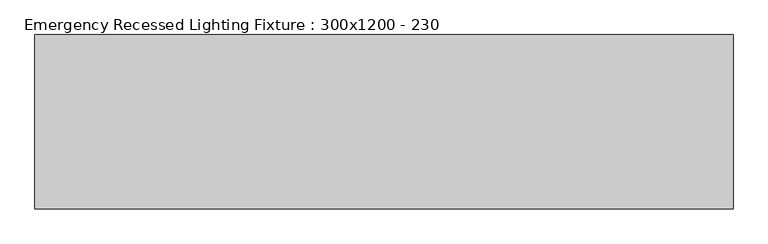
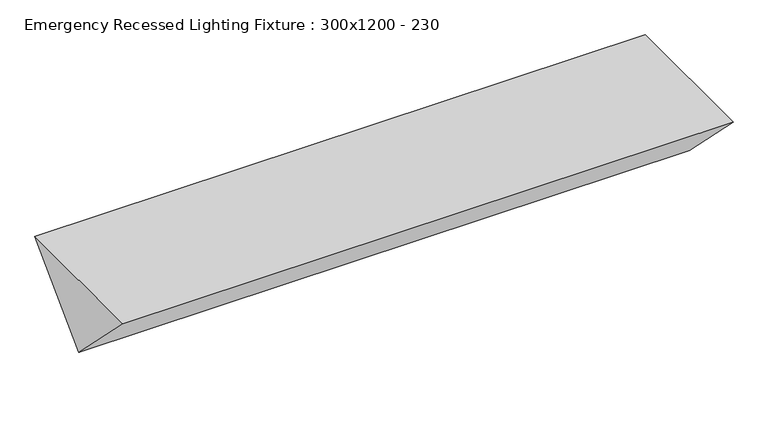
"""IFC4 building model written with IfcOpenShell, lengths in millimetres: light fixture geometry, Emergency Recessed Lighting Fixture : 300x1200 - 230."""

from ifc_helpers import new_model, si_unit, frame, origin, place, context, project, spatial, polyline, outline, extrude, source, transform, mapped, element, save


def emergency_recessed_lighting_fixture_300x1200_230_e46e8774(model_context):
    return source(origin(), model_context, "Body", "SweptSolid", [
        extrude(outline(polyline([(-300.0, 0.0), (0.0, 0.0), (-150.0, -150.0), (-300.0, 0.0)])), frame((0.0, 0.0, 0.0), z_axis=(1.0, 0.0, 0.0), x_axis=(0.0, 1.0, 0.0)), (0.0, 0.0, 1.0), 1200.0),
    ])


if __name__ == "__main__":
    model = new_model("IFC4")
    model_context = context("Model", 3, world=origin())
    ifc_project = project(units=[si_unit("LENGTHUNIT", "METRE", prefix="MILLI")], contexts=[model_context])
    site = spatial("IfcSite", under=ifc_project)
    building = spatial("IfcBuilding", under=site)
    placement = place(None, origin())
    emergency_recessed_lighting_fixture_300x1200_230_shape = emergency_recessed_lighting_fixture_300x1200_230_e46e8774(model_context)
    element("IfcLightFixture", 1, ObjectType="Emergency Recessed Lighting Fixture : 300x1200 - 230", at=placement, inside=building, context=model_context, shape_type="MappedRepresentation", body=[
        mapped(emergency_recessed_lighting_fixture_300x1200_230_shape, transform((0.0, 0.0, 0.0), x_axis=(1.0, 0.0, 0.0), y_axis=(0.0, 1.0, 0.0), z_axis=(0.0, 0.0, 1.0))),
    ])
    save(model, "model.ifc")

# Revit data of these elements
# Type "Emergency Recessed Lighting Fixture : 300x1200 - 230"
#   Photometric Web File = "1x42A12.ies"
#   Width = 300 mm
#   Wattage = 64 W
#   built-in parameter 1150110 = 1 (stored number, unit not read)
#   built-in parameter 1150109 = 1 (stored number, unit not read)
#   built-in parameter 1150113 = 1 (stored number, unit not read)
#   Tilt Angle = -90.00°
#   Normal Voltage = 230 V
#   Lumens = 5699.84 lm
#   built-in parameter 1114217 = 0.88 (stored number, unit not read)
#   built-in parameter 1150115 = 1 (stored number, unit not read)
#   built-in parameter 1150105 = 453.579 (stored number, unit not read)
#   Length = 1200 mm
#   built-in parameter 1150112 = 1 (stored number, unit not read)
#   built-in parameter 1150114 = 1 (stored number, unit not read)
#   built-in parameter 1150107 = 4230 (stored number, unit not read)
#   built-in parameter 1150106 = 4.53579 (stored number, unit not read)
#   Emit from Rectangle Width = 300 mm
#   Emit from Rectangle Length = 1200 mm
#   Emergency Voltage = 230 V
#   Emergency Load = 32 VA
#   built-in parameter 1150104 = 8.27394 (stored number, unit not read)
#   Depth = 150 mm
#   Default Elevation = 2000 mm
#   built-in parameter 1114218 = 0.88 (stored number, unit not read)
#   built-in parameter 1150133 = 10 (stored number, unit not read)
#   Apparent Load = 64 VA
#   built-in parameter 1150134 = 8
#   built-in parameter 1150137 = 1
#   Color Filter = 16777215
#   built-in parameter 1140040 [instance default] = 1
#   Load Classification = Lighting - Dwelling Unit
#   Emit Shape Visible in Rendering = no
#   Dimming Lamp Color Temperature Shift = (empty or 0)
#   Assembly Code = ""
